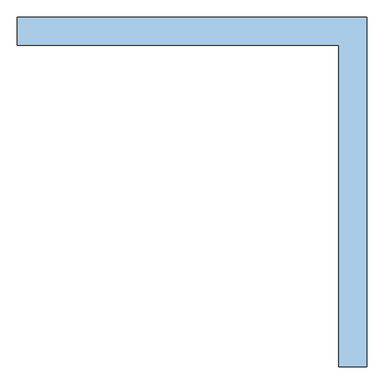
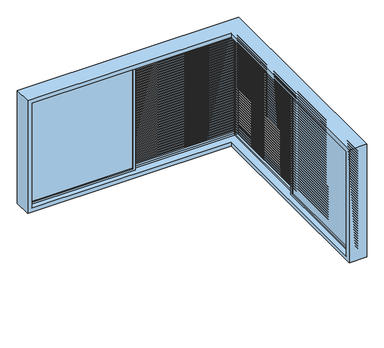
"""IFC4 building model written with IfcOpenShell, lengths in millimetres: window geometry, .CC_ND 300_JANELA DE CANTO_6 FOLHAS DE CORRER_VENEZIANA_VIDRO : 2.50F X 2.50E X 1.35H."""

from ifc_helpers import new_model, si_unit, frame, origin, place, context, project, spatial, polyline, outline, extrude, faceted_brep, source, transform, mapped, element, save


def window_869adda8(model_context):
    return source(origin(), model_context, "Body", "SolidModel", [
        extrude(outline(polyline([(2110.1282051, 1161.2), (2110.1282051, 1166.2), (2145.1282051, 1141.2), (2145.1282051, 1136.2), (2110.1282051, 1161.2)])), frame((0.0, -1170.6, 0.0), z_axis=(0.0, 1.0, 0.0), x_axis=(0.0, 0.0, 1.0)), (0.0, 0.0, 1.0), 1130.6),
        extrude(outline(polyline([(2080.2564103, 1161.2), (2080.2564103, 1166.2), (2115.2564103, 1141.2), (2115.2564103, 1136.2), (2080.2564103, 1161.2)])), frame((0.0, -1170.6, 0.0), z_axis=(0.0, 1.0, 0.0), x_axis=(0.0, 0.0, 1.0)), (0.0, 0.0, 1.0), 1130.6),
        extrude(outline(polyline([(2050.3846154, 1161.2), (2050.3846154, 1166.2), (2085.3846154, 1141.2), (2085.3846154, 1136.2), (2050.3846154, 1161.2)])), frame((0.0, -1170.6, 0.0), z_axis=(0.0, 1.0, 0.0), x_axis=(0.0, 0.0, 1.0)), (0.0, 0.0, 1.0), 1130.6),
        extrude(outline(polyline([(2020.5128205, 1161.2), (2020.5128205, 1166.2), (2055.5128205, 1141.2), (2055.5128205, 1136.2), (2020.5128205, 1161.2)])), frame((0.0, -1170.6, 0.0), z_axis=(0.0, 1.0, 0.0), x_axis=(0.0, 0.0, 1.0)), (0.0, 0.0, 1.0), 1130.6),
        extrude(outline(polyline([(1990.6410256, 1161.2), (1990.6410256, 1166.2), (2025.6410256, 1141.2), (2025.6410256, 1136.2), (1990.6410256, 1161.2)])), frame((0.0, -1170.6, 0.0), z_axis=(0.0, 1.0, 0.0), x_axis=(0.0, 0.0, 1.0)), (0.0, 0.0, 1.0), 1130.6),
        extrude(outline(polyline([(1960.7692308, 1161.2), (1960.7692308, 1166.2), (1995.7692308, 1141.2), (1995.7692308, 1136.2), (1960.7692308, 1161.2)])), frame((0.0, -1170.6, 0.0), z_axis=(0.0, 1.0, 0.0), x_axis=(0.0, 0.0, 1.0)), (0.0, 0.0, 1.0), 1130.6),
        extrude(outline(polyline([(1930.8974359, 1161.2), (1930.8974359, 1166.2), (1965.8974359, 1141.2), (1965.8974359, 1136.2), (1930.8974359, 1161.2)])), frame((0.0, -1170.6, 0.0), z_axis=(0.0, 1.0, 0.0), x_axis=(0.0, 0.0, 1.0)), (0.0, 0.0, 1.0), 1130.6),
        extrude(outline(polyline([(1901.025641, 1161.2), (1901.025641, 1166.2), (1936.025641, 1141.2), (1936.025641, 1136.2), (1901.025641, 1161.2)])), frame((0.0, -1170.6, 0.0), z_axis=(0.0, 1.0, 0.0), x_axis=(0.0, 0.0, 1.0)), (0.0, 0.0, 1.0), 1130.6),
        extrude(outline(polyline([(1871.1538462, 1161.2), (1871.1538462, 1166.2), (1906.1538462, 1141.2), (1906.1538462, 1136.2), (1871.1538462, 1161.2)])), frame((0.0, -1170.6, 0.0), z_axis=(0.0, 1.0, 0.0), x_axis=(0.0, 0.0, 1.0)), (0.0, 0.0, 1.0), 1130.6),
        extrude(outline(polyline([(1841.2820513, 1161.2), (1841.2820513, 1166.2), (1876.2820513, 1141.2), (1876.2820513, 1136.2), (1841.2820513, 1161.2)])), frame((0.0, -1170.6, 0.0), z_axis=(0.0, 1.0, 0.0), x_axis=(0.0, 0.0, 1.0)), (0.0, 0.0, 1.0), 1130.6),
        extrude(outline(polyline([(1811.4102564, 1161.2), (1811.4102564, 1166.2), (1846.4102564, 1141.2), (1846.4102564, 1136.2), (1811.4102564, 1161.2)])), frame((0.0, -1170.6, 0.0), z_axis=(0.0, 1.0, 0.0), x_axis=(0.0, 0.0, 1.0)), (0.0, 0.0, 1.0), 1130.6),
        extrude(outline(polyline([(1781.5384615, 1161.2), (1781.5384615, 1166.2), (1816.5384615, 1141.2), (1816.5384615, 1136.2), (1781.5384615, 1161.2)])), frame((0.0, -1170.6, 0.0), z_axis=(0.0, 1.0, 0.0), x_axis=(0.0, 0.0, 1.0)), (0.0, 0.0, 1.0), 1130.6),
        extrude(outline(polyline([(1751.6666667, 1161.2), (1751.6666667, 1166.2), (1786.6666667, 1141.2), (1786.6666667, 1136.2), (1751.6666667, 1161.2)])), frame((0.0, -1170.6, 0.0), z_axis=(0.0, 1.0, 0.0), x_axis=(0.0, 0.0, 1.0)), (0.0, 0.0, 1.0), 1130.6),
        extrude(outline(polyline([(1721.7948718, 1161.2), (1721.7948718, 1166.2), (1756.7948718, 1141.2), (1756.7948718, 1136.2), (1721.7948718, 1161.2)])), frame((0.0, -1170.6, 0.0), z_axis=(0.0, 1.0, 0.0), x_axis=(0.0, 0.0, 1.0)), (0.0, 0.0, 1.0), 1130.6),
        extrude(outline(polyline([(1691.9230769, 1161.2), (1691.9230769, 1166.2), (1726.9230769, 1141.2), (1726.9230769, 1136.2), (1691.9230769, 1161.2)])), frame((0.0, -1170.6, 0.0), z_axis=(0.0, 1.0, 0.0), x_axis=(0.0, 0.0, 1.0)), (0.0, 0.0, 1.0), 1130.6),
        extrude(outline(polyline([(1662.0512821, 1161.2), (1662.0512821, 1166.2), (1697.0512821, 1141.2), (1697.0512821, 1136.2), (1662.0512821, 1161.2)])), frame((0.0, -1170.6, 0.0), z_axis=(0.0, 1.0, 0.0), x_axis=(0.0, 0.0, 1.0)), (0.0, 0.0, 1.0), 1130.6),
        extrude(outline(polyline([(1632.1794872, 1161.2), (1632.1794872, 1166.2), (1667.1794872, 1141.2), (1667.1794872, 1136.2), (1632.1794872, 1161.2)])), frame((0.0, -1170.6, 0.0), z_axis=(0.0, 1.0, 0.0), x_axis=(0.0, 0.0, 1.0)), (0.0, 0.0, 1.0), 1130.6),
        extrude(outline(polyline([(1602.3076923, 1161.2), (1602.3076923, 1166.2), (1637.3076923, 1141.2), (1637.3076923, 1136.2), (1602.3076923, 1161.2)])), frame((0.0, -1170.6, 0.0), z_axis=(0.0, 1.0, 0.0), x_axis=(0.0, 0.0, 1.0)), (0.0, 0.0, 1.0), 1130.6),
        extrude(outline(polyline([(1572.4358974, 1161.2), (1572.4358974, 1166.2), (1607.4358974, 1141.2), (1607.4358974, 1136.2), (1572.4358974, 1161.2)])), frame((0.0, -1170.6, 0.0), z_axis=(0.0, 1.0, 0.0), x_axis=(0.0, 0.0, 1.0)), (0.0, 0.0, 1.0), 1130.6),
        extrude(outline(polyline([(1542.5641026, 1161.2), (1542.5641026, 1166.2), (1577.5641026, 1141.2), (1577.5641026, 1136.2), (1542.5641026, 1161.2)])), frame((0.0, -1170.6, 0.0), z_axis=(0.0, 1.0, 0.0), x_axis=(0.0, 0.0, 1.0)), (0.0, 0.0, 1.0), 1130.6),
        extrude(outline(polyline([(1512.6923077, 1161.2), (1512.6923077, 1166.2), (1547.6923077, 1141.2), (1547.6923077, 1136.2), (1512.6923077, 1161.2)])), frame((0.0, -1170.6, 0.0), z_axis=(0.0, 1.0, 0.0), x_axis=(0.0, 0.0, 1.0)), (0.0, 0.0, 1.0), 1130.6),
        extrude(outline(polyline([(1482.8205128, 1161.2), (1482.8205128, 1166.2), (1517.8205128, 1141.2), (1517.8205128, 1136.2), (1482.8205128, 1161.2)])), frame((0.0, -1170.6, 0.0), z_axis=(0.0, 1.0, 0.0), x_axis=(0.0, 0.0, 1.0)), (0.0, 0.0, 1.0), 1130.6),
        extrude(outline(polyline([(1452.9487179, 1161.2), (1452.9487179, 1166.2), (1487.9487179, 1141.2), (1487.9487179, 1136.2), (1452.9487179, 1161.2)])), frame((0.0, -1170.6, 0.0), z_axis=(0.0, 1.0, 0.0), x_axis=(0.0, 0.0, 1.0)), (0.0, 0.0, 1.0), 1130.6),
        extrude(outline(polyline([(1423.0769231, 1161.2), (1423.0769231, 1166.2), (1458.0769231, 1141.2), (1458.0769231, 1136.2), (1423.0769231, 1161.2)])), frame((0.0, -1170.6, 0.0), z_axis=(0.0, 1.0, 0.0), x_axis=(0.0, 0.0, 1.0)), (0.0, 0.0, 1.0), 1130.6),
        extrude(outline(polyline([(1393.2051282, 1161.2), (1393.2051282, 1166.2), (1428.2051282, 1141.2), (1428.2051282, 1136.2), (1393.2051282, 1161.2)])), frame((0.0, -1170.6, 0.0), z_axis=(0.0, 1.0, 0.0), x_axis=(0.0, 0.0, 1.0)), (0.0, 0.0, 1.0), 1130.6),
        extrude(outline(polyline([(1363.3333333, 1161.2), (1363.3333333, 1166.2), (1398.3333333, 1141.2), (1398.3333333, 1136.2), (1363.3333333, 1161.2)])), frame((0.0, -1170.6, 0.0), z_axis=(0.0, 1.0, 0.0), x_axis=(0.0, 0.0, 1.0)), (0.0, 0.0, 1.0), 1130.6),
        extrude(outline(polyline([(1333.4615385, 1161.2), (1333.4615385, 1166.2), (1368.4615385, 1141.2), (1368.4615385, 1136.2), (1333.4615385, 1161.2)])), frame((0.0, -1170.6, 0.0), z_axis=(0.0, 1.0, 0.0), x_axis=(0.0, 0.0, 1.0)), (0.0, 0.0, 1.0), 1130.6),
        extrude(outline(polyline([(1303.5897436, 1161.2), (1303.5897436, 1166.2), (1338.5897436, 1141.2), (1338.5897436, 1136.2), (1303.5897436, 1161.2)])), frame((0.0, -1170.6, 0.0), z_axis=(0.0, 1.0, 0.0), x_axis=(0.0, 0.0, 1.0)), (0.0, 0.0, 1.0), 1130.6),
        extrude(outline(polyline([(1273.7179487, 1161.2), (1273.7179487, 1166.2), (1308.7179487, 1141.2), (1308.7179487, 1136.2), (1273.7179487, 1161.2)])), frame((0.0, -1170.6, 0.0), z_axis=(0.0, 1.0, 0.0), x_axis=(0.0, 0.0, 1.0)), (0.0, 0.0, 1.0), 1130.6),
        extrude(outline(polyline([(1243.8461538, 1161.2), (1243.8461538, 1166.2), (1278.8461538, 1141.2), (1278.8461538, 1136.2), (1243.8461538, 1161.2)])), frame((0.0, -1170.6, 0.0), z_axis=(0.0, 1.0, 0.0), x_axis=(0.0, 0.0, 1.0)), (0.0, 0.0, 1.0), 1130.6),
        extrude(outline(polyline([(1213.974359, 1161.2), (1213.974359, 1166.2), (1248.974359, 1141.2), (1248.974359, 1136.2), (1213.974359, 1161.2)])), frame((0.0, -1170.6, 0.0), z_axis=(0.0, 1.0, 0.0), x_axis=(0.0, 0.0, 1.0)), (0.0, 0.0, 1.0), 1130.6),
        extrude(outline(polyline([(1184.1025641, 1161.2), (1184.1025641, 1166.2), (1219.1025641, 1141.2), (1219.1025641, 1136.2), (1184.1025641, 1161.2)])), frame((0.0, -1170.6, 0.0), z_axis=(0.0, 1.0, 0.0), x_axis=(0.0, 0.0, 1.0)), (0.0, 0.0, 1.0), 1130.6),
        extrude(outline(polyline([(1154.2307692, 1161.2), (1154.2307692, 1166.2), (1189.2307692, 1141.2), (1189.2307692, 1136.2), (1154.2307692, 1161.2)])), frame((0.0, -1170.6, 0.0), z_axis=(0.0, 1.0, 0.0), x_axis=(0.0, 0.0, 1.0)), (0.0, 0.0, 1.0), 1130.6),
        extrude(outline(polyline([(1124.3589744, 1161.2), (1124.3589744, 1166.2), (1159.3589744, 1141.2), (1159.3589744, 1136.2), (1124.3589744, 1161.2)])), frame((0.0, -1170.6, 0.0), z_axis=(0.0, 1.0, 0.0), x_axis=(0.0, 0.0, 1.0)), (0.0, 0.0, 1.0), 1130.6),
        extrude(outline(polyline([(1094.4871795, 1161.2), (1094.4871795, 1166.2), (1129.4871795, 1141.2), (1129.4871795, 1136.2), (1094.4871795, 1161.2)])), frame((0.0, -1170.6, 0.0), z_axis=(0.0, 1.0, 0.0), x_axis=(0.0, 0.0, 1.0)), (0.0, 0.0, 1.0), 1130.6),
        extrude(outline(polyline([(1064.6153846, 1161.2), (1064.6153846, 1166.2), (1099.6153846, 1141.2), (1099.6153846, 1136.2), (1064.6153846, 1161.2)])), frame((0.0, -1170.6, 0.0), z_axis=(0.0, 1.0, 0.0), x_axis=(0.0, 0.0, 1.0)), (0.0, 0.0, 1.0), 1130.6),
        extrude(outline(polyline([(1034.7435897, 1161.2), (1034.7435897, 1166.2), (1069.7435897, 1141.2), (1069.7435897, 1136.2), (1034.7435897, 1161.2)])), frame((0.0, -1170.6, 0.0), z_axis=(0.0, 1.0, 0.0), x_axis=(0.0, 0.0, 1.0)), (0.0, 0.0, 1.0), 1130.6),
        extrude(outline(polyline([(1004.8717949, 1161.2), (1004.8717949, 1166.2), (1039.8717949, 1141.2), (1039.8717949, 1136.2), (1004.8717949, 1161.2)])), frame((0.0, -1170.6, 0.0), z_axis=(0.0, 1.0, 0.0), x_axis=(0.0, 0.0, 1.0)), (0.0, 0.0, 1.0), 1130.6),
        extrude(outline(polyline([(2140.0, 1161.2), (2140.0, 1166.2), (2175.0, 1141.2), (2175.0, 1136.2), (2140.0, 1161.2)])), frame((0.0, -1170.6, 0.0), z_axis=(0.0, 1.0, 0.0), x_axis=(0.0, 0.0, 1.0)), (0.0, 0.0, 1.0), 1130.6),
        extrude(outline(polyline([(975.0, 1161.2), (975.0, 1166.2), (1010.0, 1141.2), (1010.0, 1136.2), (975.0, 1161.2)])), frame((0.0, -1170.6, 0.0), z_axis=(0.0, 1.0, 0.0), x_axis=(0.0, 0.0, 1.0)), (0.0, 0.0, 1.0), 1130.6),
        extrude(outline(polyline([(-15.0, 2200.0), (-15.0, 950.0), (-1195.6, 950.0), (-1195.6, 2200.0), (-15.0, 2200.0)]), holes=[polyline([(-40.0, 2175.0), (-1170.6, 2175.0), (-1170.6, 975.0), (-40.0, 975.0), (-40.0, 2175.0)])]), frame((1136.2, 0.0, 0.0), z_axis=(1.0, 0.0, 0.0), x_axis=(0.0, 1.0, 0.0)), (0.0, 0.0, 1.0), 30.0),
        extrude(outline(polyline([(2110.1282051, 1191.2), (2110.1282051, 1196.2), (2145.1282051, 1171.2), (2145.1282051, 1166.2), (2110.1282051, 1191.2)])), frame((0.0, -2326.2, 0.0), z_axis=(0.0, 1.0, 0.0), x_axis=(0.0, 0.0, 1.0)), (0.0, 0.0, 1.0), 1130.6),
        extrude(outline(polyline([(2080.2564103, 1191.2), (2080.2564103, 1196.2), (2115.2564103, 1171.2), (2115.2564103, 1166.2), (2080.2564103, 1191.2)])), frame((0.0, -2326.2, 0.0), z_axis=(0.0, 1.0, 0.0), x_axis=(0.0, 0.0, 1.0)), (0.0, 0.0, 1.0), 1130.6),
        extrude(outline(polyline([(2050.3846154, 1191.2), (2050.3846154, 1196.2), (2085.3846154, 1171.2), (2085.3846154, 1166.2), (2050.3846154, 1191.2)])), frame((0.0, -2326.2, 0.0), z_axis=(0.0, 1.0, 0.0), x_axis=(0.0, 0.0, 1.0)), (0.0, 0.0, 1.0), 1130.6),
        extrude(outline(polyline([(2020.5128205, 1191.2), (2020.5128205, 1196.2), (2055.5128205, 1171.2), (2055.5128205, 1166.2), (2020.5128205, 1191.2)])), frame((0.0, -2326.2, 0.0), z_axis=(0.0, 1.0, 0.0), x_axis=(0.0, 0.0, 1.0)), (0.0, 0.0, 1.0), 1130.6),
        extrude(outline(polyline([(1990.6410256, 1191.2), (1990.6410256, 1196.2), (2025.6410256, 1171.2), (2025.6410256, 1166.2), (1990.6410256, 1191.2)])), frame((0.0, -2326.2, 0.0), z_axis=(0.0, 1.0, 0.0), x_axis=(0.0, 0.0, 1.0)), (0.0, 0.0, 1.0), 1130.6),
        extrude(outline(polyline([(1960.7692308, 1191.2), (1960.7692308, 1196.2), (1995.7692308, 1171.2), (1995.7692308, 1166.2), (1960.7692308, 1191.2)])), frame((0.0, -2326.2, 0.0), z_axis=(0.0, 1.0, 0.0), x_axis=(0.0, 0.0, 1.0)), (0.0, 0.0, 1.0), 1130.6),
        extrude(outline(polyline([(1930.8974359, 1191.2), (1930.8974359, 1196.2), (1965.8974359, 1171.2), (1965.8974359, 1166.2), (1930.8974359, 1191.2)])), frame((0.0, -2326.2, 0.0), z_axis=(0.0, 1.0, 0.0), x_axis=(0.0, 0.0, 1.0)), (0.0, 0.0, 1.0), 1130.6),
        extrude(outline(polyline([(1901.025641, 1191.2), (1901.025641, 1196.2), (1936.025641, 1171.2), (1936.025641, 1166.2), (1901.025641, 1191.2)])), frame((0.0, -2326.2, 0.0), z_axis=(0.0, 1.0, 0.0), x_axis=(0.0, 0.0, 1.0)), (0.0, 0.0, 1.0), 1130.6),
        extrude(outline(polyline([(1871.1538462, 1191.2), (1871.1538462, 1196.2), (1906.1538462, 1171.2), (1906.1538462, 1166.2), (1871.1538462, 1191.2)])), frame((0.0, -2326.2, 0.0), z_axis=(0.0, 1.0, 0.0), x_axis=(0.0, 0.0, 1.0)), (0.0, 0.0, 1.0), 1130.6),
        extrude(outline(polyline([(1841.2820513, 1191.2), (1841.2820513, 1196.2), (1876.2820513, 1171.2), (1876.2820513, 1166.2), (1841.2820513, 1191.2)])), frame((0.0, -2326.2, 0.0), z_axis=(0.0, 1.0, 0.0), x_axis=(0.0, 0.0, 1.0)), (0.0, 0.0, 1.0), 1130.6),
        extrude(outline(polyline([(1811.4102564, 1191.2), (1811.4102564, 1196.2), (1846.4102564, 1171.2), (1846.4102564, 1166.2), (1811.4102564, 1191.2)])), frame((0.0, -2326.2, 0.0), z_axis=(0.0, 1.0, 0.0), x_axis=(0.0, 0.0, 1.0)), (0.0, 0.0, 1.0), 1130.6),
        extrude(outline(polyline([(1781.5384615, 1191.2), (1781.5384615, 1196.2), (1816.5384615, 1171.2), (1816.5384615, 1166.2), (1781.5384615, 1191.2)])), frame((0.0, -2326.2, 0.0), z_axis=(0.0, 1.0, 0.0), x_axis=(0.0, 0.0, 1.0)), (0.0, 0.0, 1.0), 1130.6),
        extrude(outline(polyline([(1751.6666667, 1191.2), (1751.6666667, 1196.2), (1786.6666667, 1171.2), (1786.6666667, 1166.2), (1751.6666667, 1191.2)])), frame((0.0, -2326.2, 0.0), z_axis=(0.0, 1.0, 0.0), x_axis=(0.0, 0.0, 1.0)), (0.0, 0.0, 1.0), 1130.6),
        extrude(outline(polyline([(1721.7948718, 1191.2), (1721.7948718, 1196.2), (1756.7948718, 1171.2), (1756.7948718, 1166.2), (1721.7948718, 1191.2)])), frame((0.0, -2326.2, 0.0), z_axis=(0.0, 1.0, 0.0), x_axis=(0.0, 0.0, 1.0)), (0.0, 0.0, 1.0), 1130.6),
        extrude(outline(polyline([(1691.9230769, 1191.2), (1691.9230769, 1196.2), (1726.9230769, 1171.2), (1726.9230769, 1166.2), (1691.9230769, 1191.2)])), frame((0.0, -2326.2, 0.0), z_axis=(0.0, 1.0, 0.0), x_axis=(0.0, 0.0, 1.0)), (0.0, 0.0, 1.0), 1130.6),
        extrude(outline(polyline([(1662.0512821, 1191.2), (1662.0512821, 1196.2), (1697.0512821, 1171.2), (1697.0512821, 1166.2), (1662.0512821, 1191.2)])), frame((0.0, -2326.2, 0.0), z_axis=(0.0, 1.0, 0.0), x_axis=(0.0, 0.0, 1.0)), (0.0, 0.0, 1.0), 1130.6),
        extrude(outline(polyline([(1632.1794872, 1191.2), (1632.1794872, 1196.2), (1667.1794872, 1171.2), (1667.1794872, 1166.2), (1632.1794872, 1191.2)])), frame((0.0, -2326.2, 0.0), z_axis=(0.0, 1.0, 0.0), x_axis=(0.0, 0.0, 1.0)), (0.0, 0.0, 1.0), 1130.6),
        extrude(outline(polyline([(1602.3076923, 1191.2), (1602.3076923, 1196.2), (1637.3076923, 1171.2), (1637.3076923, 1166.2), (1602.3076923, 1191.2)])), frame((0.0, -2326.2, 0.0), z_axis=(0.0, 1.0, 0.0), x_axis=(0.0, 0.0, 1.0)), (0.0, 0.0, 1.0), 1130.6),
        extrude(outline(polyline([(1572.4358974, 1191.2), (1572.4358974, 1196.2), (1607.4358974, 1171.2), (1607.4358974, 1166.2), (1572.4358974, 1191.2)])), frame((0.0, -2326.2, 0.0), z_axis=(0.0, 1.0, 0.0), x_axis=(0.0, 0.0, 1.0)), (0.0, 0.0, 1.0), 1130.6),
        extrude(outline(polyline([(1542.5641026, 1191.2), (1542.5641026, 1196.2), (1577.5641026, 1171.2), (1577.5641026, 1166.2), (1542.5641026, 1191.2)])), frame((0.0, -2326.2, 0.0), z_axis=(0.0, 1.0, 0.0), x_axis=(0.0, 0.0, 1.0)), (0.0, 0.0, 1.0), 1130.6),
        extrude(outline(polyline([(1512.6923077, 1191.2), (1512.6923077, 1196.2), (1547.6923077, 1171.2), (1547.6923077, 1166.2), (1512.6923077, 1191.2)])), frame((0.0, -2326.2, 0.0), z_axis=(0.0, 1.0, 0.0), x_axis=(0.0, 0.0, 1.0)), (0.0, 0.0, 1.0), 1130.6),
        extrude(outline(polyline([(1482.8205128, 1191.2), (1482.8205128, 1196.2), (1517.8205128, 1171.2), (1517.8205128, 1166.2), (1482.8205128, 1191.2)])), frame((0.0, -2326.2, 0.0), z_axis=(0.0, 1.0, 0.0), x_axis=(0.0, 0.0, 1.0)), (0.0, 0.0, 1.0), 1130.6),
        extrude(outline(polyline([(1452.9487179, 1191.2), (1452.9487179, 1196.2), (1487.9487179, 1171.2), (1487.9487179, 1166.2), (1452.9487179, 1191.2)])), frame((0.0, -2326.2, 0.0), z_axis=(0.0, 1.0, 0.0), x_axis=(0.0, 0.0, 1.0)), (0.0, 0.0, 1.0), 1130.6),
        extrude(outline(polyline([(1423.0769231, 1191.2), (1423.0769231, 1196.2), (1458.0769231, 1171.2), (1458.0769231, 1166.2), (1423.0769231, 1191.2)])), frame((0.0, -2326.2, 0.0), z_axis=(0.0, 1.0, 0.0), x_axis=(0.0, 0.0, 1.0)), (0.0, 0.0, 1.0), 1130.6),
        extrude(outline(polyline([(1393.2051282, 1191.2), (1393.2051282, 1196.2), (1428.2051282, 1171.2), (1428.2051282, 1166.2), (1393.2051282, 1191.2)])), frame((0.0, -2326.2, 0.0), z_axis=(0.0, 1.0, 0.0), x_axis=(0.0, 0.0, 1.0)), (0.0, 0.0, 1.0), 1130.6),
        extrude(outline(polyline([(1363.3333333, 1191.2), (1363.3333333, 1196.2), (1398.3333333, 1171.2), (1398.3333333, 1166.2), (1363.3333333, 1191.2)])), frame((0.0, -2326.2, 0.0), z_axis=(0.0, 1.0, 0.0), x_axis=(0.0, 0.0, 1.0)), (0.0, 0.0, 1.0), 1130.6),
        extrude(outline(polyline([(1333.4615385, 1191.2), (1333.4615385, 1196.2), (1368.4615385, 1171.2), (1368.4615385, 1166.2), (1333.4615385, 1191.2)])), frame((0.0, -2326.2, 0.0), z_axis=(0.0, 1.0, 0.0), x_axis=(0.0, 0.0, 1.0)), (0.0, 0.0, 1.0), 1130.6),
        extrude(outline(polyline([(1303.5897436, 1191.2), (1303.5897436, 1196.2), (1338.5897436, 1171.2), (1338.5897436, 1166.2), (1303.5897436, 1191.2)])), frame((0.0, -2326.2, 0.0), z_axis=(0.0, 1.0, 0.0), x_axis=(0.0, 0.0, 1.0)), (0.0, 0.0, 1.0), 1130.6),
        extrude(outline(polyline([(1273.7179487, 1191.2), (1273.7179487, 1196.2), (1308.7179487, 1171.2), (1308.7179487, 1166.2), (1273.7179487, 1191.2)])), frame((0.0, -2326.2, 0.0), z_axis=(0.0, 1.0, 0.0), x_axis=(0.0, 0.0, 1.0)), (0.0, 0.0, 1.0), 1130.6),
        extrude(outline(polyline([(1243.8461538, 1191.2), (1243.8461538, 1196.2), (1278.8461538, 1171.2), (1278.8461538, 1166.2), (1243.8461538, 1191.2)])), frame((0.0, -2326.2, 0.0), z_axis=(0.0, 1.0, 0.0), x_axis=(0.0, 0.0, 1.0)), (0.0, 0.0, 1.0), 1130.6),
        extrude(outline(polyline([(1213.974359, 1191.2), (1213.974359, 1196.2), (1248.974359, 1171.2), (1248.974359, 1166.2), (1213.974359, 1191.2)])), frame((0.0, -2326.2, 0.0), z_axis=(0.0, 1.0, 0.0), x_axis=(0.0, 0.0, 1.0)), (0.0, 0.0, 1.0), 1130.6),
        extrude(outline(polyline([(1184.1025641, 1191.2), (1184.1025641, 1196.2), (1219.1025641, 1171.2), (1219.1025641, 1166.2), (1184.1025641, 1191.2)])), frame((0.0, -2326.2, 0.0), z_axis=(0.0, 1.0, 0.0), x_axis=(0.0, 0.0, 1.0)), (0.0, 0.0, 1.0), 1130.6),
        extrude(outline(polyline([(1154.2307692, 1191.2), (1154.2307692, 1196.2), (1189.2307692, 1171.2), (1189.2307692, 1166.2), (1154.2307692, 1191.2)])), frame((0.0, -2326.2, 0.0), z_axis=(0.0, 1.0, 0.0), x_axis=(0.0, 0.0, 1.0)), (0.0, 0.0, 1.0), 1130.6),
        extrude(outline(polyline([(1124.3589744, 1191.2), (1124.3589744, 1196.2), (1159.3589744, 1171.2), (1159.3589744, 1166.2), (1124.3589744, 1191.2)])), frame((0.0, -2326.2, 0.0), z_axis=(0.0, 1.0, 0.0), x_axis=(0.0, 0.0, 1.0)), (0.0, 0.0, 1.0), 1130.6),
        extrude(outline(polyline([(1094.4871795, 1191.2), (1094.4871795, 1196.2), (1129.4871795, 1171.2), (1129.4871795, 1166.2), (1094.4871795, 1191.2)])), frame((0.0, -2326.2, 0.0), z_axis=(0.0, 1.0, 0.0), x_axis=(0.0, 0.0, 1.0)), (0.0, 0.0, 1.0), 1130.6),
        extrude(outline(polyline([(1064.6153846, 1191.2), (1064.6153846, 1196.2), (1099.6153846, 1171.2), (1099.6153846, 1166.2), (1064.6153846, 1191.2)])), frame((0.0, -2326.2, 0.0), z_axis=(0.0, 1.0, 0.0), x_axis=(0.0, 0.0, 1.0)), (0.0, 0.0, 1.0), 1130.6),
        extrude(outline(polyline([(1034.7435897, 1191.2), (1034.7435897, 1196.2), (1069.7435897, 1171.2), (1069.7435897, 1166.2), (1034.7435897, 1191.2)])), frame((0.0, -2326.2, 0.0), z_axis=(0.0, 1.0, 0.0), x_axis=(0.0, 0.0, 1.0)), (0.0, 0.0, 1.0), 1130.6),
        extrude(outline(polyline([(1004.8717949, 1191.2), (1004.8717949, 1196.2), (1039.8717949, 1171.2), (1039.8717949, 1166.2), (1004.8717949, 1191.2)])), frame((0.0, -2326.2, 0.0), z_axis=(0.0, 1.0, 0.0), x_axis=(0.0, 0.0, 1.0)), (0.0, 0.0, 1.0), 1130.6),
        extrude(outline(polyline([(2140.0, 1191.2), (2140.0, 1196.2), (2175.0, 1171.2), (2175.0, 1166.2), (2140.0, 1191.2)])), frame((0.0, -2326.2, 0.0), z_axis=(0.0, 1.0, 0.0), x_axis=(0.0, 0.0, 1.0)), (0.0, 0.0, 1.0), 1130.6),
        extrude(outline(polyline([(975.0, 1191.2), (975.0, 1196.2), (1010.0, 1171.2), (1010.0, 1166.2), (975.0, 1191.2)])), frame((0.0, -2326.2, 0.0), z_axis=(0.0, 1.0, 0.0), x_axis=(0.0, 0.0, 1.0)), (0.0, 0.0, 1.0), 1130.6),
        extrude(outline(polyline([(-1170.6, 2200.0), (-1170.6, 950.0), (-2351.2, 950.0), (-2351.2, 2200.0), (-1170.6, 2200.0)]), holes=[polyline([(-1195.6, 2175.0), (-2326.2, 2175.0), (-2326.2, 975.0), (-1195.6, 975.0), (-1195.6, 2175.0)])]), frame((1166.2, 0.0, 0.0), z_axis=(1.0, 0.0, 0.0), x_axis=(0.0, 1.0, 0.0)), (0.0, 0.0, 1.0), 30.0),
        extrude(outline(polyline([(-1170.6, 2200.0), (-1170.6, 950.0), (-2351.2, 950.0), (-2351.2, 2200.0), (-1170.6, 2200.0)]), holes=[polyline([(-1195.6, 2175.0), (-2326.2, 2175.0), (-2326.2, 975.0), (-1195.6, 975.0), (-1195.6, 2175.0)])]), frame((1106.2, 0.0, 0.0), z_axis=(1.0, 0.0, 0.0), x_axis=(0.0, 1.0, 0.0)), (0.0, 0.0, 1.0), 30.0),
        extrude(outline(polyline([(1117.2, -1195.6), (1125.2, -1195.6), (1125.2, -2326.2), (1117.2, -2326.2), (1117.2, -1195.6)])), frame((0.0, 0.0, 975.0), z_axis=(0.0, 0.0, 1.0), x_axis=(1.0, 0.0, 0.0)), (0.0, 0.0, 1.0), 1200.0),
        extrude(outline(polyline([(2200.0, -4.4), (2200.0, -1200.0), (950.0, -1200.0), (950.0, -4.4), (2200.0, -4.4)]), holes=[polyline([(2175.0, -29.4), (975.0, -29.4), (975.0, -1175.0), (2175.0, -1175.0), (2175.0, -29.4)])]), frame((0.0, -45.0, 0.0), z_axis=(0.0, 1.0, 0.0), x_axis=(0.0, 0.0, 1.0)), (0.0, 0.0, 1.0), 30.0),
        extrude(outline(polyline([(-29.4, -26.0), (-29.4, -34.0), (-1175.0, -34.0), (-1175.0, -26.0), (-29.4, -26.0)])), frame((0.0, 0.0, 975.0), z_axis=(0.0, 0.0, 1.0), x_axis=(1.0, 0.0, 0.0)), (0.0, 0.0, 1.0), 1200.0),
        extrude(outline(polyline([(10.0, 2110.1282051), (-15.0, 2145.1282051), (-10.0, 2145.1282051), (15.0, 2110.1282051), (10.0, 2110.1282051)])), frame((-4.4, 0.0, 0.0), z_axis=(1.0, 0.0, 0.0), x_axis=(0.0, 1.0, 0.0)), (0.0, 0.0, 1.0), 1145.6),
        extrude(outline(polyline([(10.0, 2080.2564103), (-15.0, 2115.2564103), (-10.0, 2115.2564103), (15.0, 2080.2564103), (10.0, 2080.2564103)])), frame((-4.4, 0.0, 0.0), z_axis=(1.0, 0.0, 0.0), x_axis=(0.0, 1.0, 0.0)), (0.0, 0.0, 1.0), 1145.6),
        extrude(outline(polyline([(10.0, 2050.3846154), (-15.0, 2085.3846154), (-10.0, 2085.3846154), (15.0, 2050.3846154), (10.0, 2050.3846154)])), frame((-4.4, 0.0, 0.0), z_axis=(1.0, 0.0, 0.0), x_axis=(0.0, 1.0, 0.0)), (0.0, 0.0, 1.0), 1145.6),
        extrude(outline(polyline([(10.0, 2020.5128205), (-15.0, 2055.5128205), (-10.0, 2055.5128205), (15.0, 2020.5128205), (10.0, 2020.5128205)])), frame((-4.4, 0.0, 0.0), z_axis=(1.0, 0.0, 0.0), x_axis=(0.0, 1.0, 0.0)), (0.0, 0.0, 1.0), 1145.6),
        extrude(outline(polyline([(10.0, 1990.6410256), (-15.0, 2025.6410256), (-10.0, 2025.6410256), (15.0, 1990.6410256), (10.0, 1990.6410256)])), frame((-4.4, 0.0, 0.0), z_axis=(1.0, 0.0, 0.0), x_axis=(0.0, 1.0, 0.0)), (0.0, 0.0, 1.0), 1145.6),
        extrude(outline(polyline([(10.0, 1960.7692308), (-15.0, 1995.7692308), (-10.0, 1995.7692308), (15.0, 1960.7692308), (10.0, 1960.7692308)])), frame((-4.4, 0.0, 0.0), z_axis=(1.0, 0.0, 0.0), x_axis=(0.0, 1.0, 0.0)), (0.0, 0.0, 1.0), 1145.6),
        extrude(outline(polyline([(10.0, 1930.8974359), (-15.0, 1965.8974359), (-10.0, 1965.8974359), (15.0, 1930.8974359), (10.0, 1930.8974359)])), frame((-4.4, 0.0, 0.0), z_axis=(1.0, 0.0, 0.0), x_axis=(0.0, 1.0, 0.0)), (0.0, 0.0, 1.0), 1145.6),
        extrude(outline(polyline([(10.0, 1901.025641), (-15.0, 1936.025641), (-10.0, 1936.025641), (15.0, 1901.025641), (10.0, 1901.025641)])), frame((-4.4, 0.0, 0.0), z_axis=(1.0, 0.0, 0.0), x_axis=(0.0, 1.0, 0.0)), (0.0, 0.0, 1.0), 1145.6),
        extrude(outline(polyline([(10.0, 1871.1538462), (-15.0, 1906.1538462), (-10.0, 1906.1538462), (15.0, 1871.1538462), (10.0, 1871.1538462)])), frame((-4.4, 0.0, 0.0), z_axis=(1.0, 0.0, 0.0), x_axis=(0.0, 1.0, 0.0)), (0.0, 0.0, 1.0), 1145.6),
        extrude(outline(polyline([(10.0, 1841.2820513), (-15.0, 1876.2820513), (-10.0, 1876.2820513), (15.0, 1841.2820513), (10.0, 1841.2820513)])), frame((-4.4, 0.0, 0.0), z_axis=(1.0, 0.0, 0.0), x_axis=(0.0, 1.0, 0.0)), (0.0, 0.0, 1.0), 1145.6),
        extrude(outline(polyline([(10.0, 1811.4102564), (-15.0, 1846.4102564), (-10.0, 1846.4102564), (15.0, 1811.4102564), (10.0, 1811.4102564)])), frame((-4.4, 0.0, 0.0), z_axis=(1.0, 0.0, 0.0), x_axis=(0.0, 1.0, 0.0)), (0.0, 0.0, 1.0), 1145.6),
        extrude(outline(polyline([(10.0, 1781.5384615), (-15.0, 1816.5384615), (-10.0, 1816.5384615), (15.0, 1781.5384615), (10.0, 1781.5384615)])), frame((-4.4, 0.0, 0.0), z_axis=(1.0, 0.0, 0.0), x_axis=(0.0, 1.0, 0.0)), (0.0, 0.0, 1.0), 1145.6),
        extrude(outline(polyline([(10.0, 1751.6666667), (-15.0, 1786.6666667), (-10.0, 1786.6666667), (15.0, 1751.6666667), (10.0, 1751.6666667)])), frame((-4.4, 0.0, 0.0), z_axis=(1.0, 0.0, 0.0), x_axis=(0.0, 1.0, 0.0)), (0.0, 0.0, 1.0), 1145.6),
        extrude(outline(polyline([(10.0, 1721.7948718), (-15.0, 1756.7948718), (-10.0, 1756.7948718), (15.0, 1721.7948718), (10.0, 1721.7948718)])), frame((-4.4, 0.0, 0.0), z_axis=(1.0, 0.0, 0.0), x_axis=(0.0, 1.0, 0.0)), (0.0, 0.0, 1.0), 1145.6),
        extrude(outline(polyline([(10.0, 1691.9230769), (-15.0, 1726.9230769), (-10.0, 1726.9230769), (15.0, 1691.9230769), (10.0, 1691.9230769)])), frame((-4.4, 0.0, 0.0), z_axis=(1.0, 0.0, 0.0), x_axis=(0.0, 1.0, 0.0)), (0.0, 0.0, 1.0), 1145.6),
        extrude(outline(polyline([(10.0, 1662.0512821), (-15.0, 1697.0512821), (-10.0, 1697.0512821), (15.0, 1662.0512821), (10.0, 1662.0512821)])), frame((-4.4, 0.0, 0.0), z_axis=(1.0, 0.0, 0.0), x_axis=(0.0, 1.0, 0.0)), (0.0, 0.0, 1.0), 1145.6),
        extrude(outline(polyline([(10.0, 1632.1794872), (-15.0, 1667.1794872), (-10.0, 1667.1794872), (15.0, 1632.1794872), (10.0, 1632.1794872)])), frame((-4.4, 0.0, 0.0), z_axis=(1.0, 0.0, 0.0), x_axis=(0.0, 1.0, 0.0)), (0.0, 0.0, 1.0), 1145.6),
        extrude(outline(polyline([(10.0, 1602.3076923), (-15.0, 1637.3076923), (-10.0, 1637.3076923), (15.0, 1602.3076923), (10.0, 1602.3076923)])), frame((-4.4, 0.0, 0.0), z_axis=(1.0, 0.0, 0.0), x_axis=(0.0, 1.0, 0.0)), (0.0, 0.0, 1.0), 1145.6),
        extrude(outline(polyline([(10.0, 1572.4358974), (-15.0, 1607.4358974), (-10.0, 1607.4358974), (15.0, 1572.4358974), (10.0, 1572.4358974)])), frame((-4.4, 0.0, 0.0), z_axis=(1.0, 0.0, 0.0), x_axis=(0.0, 1.0, 0.0)), (0.0, 0.0, 1.0), 1145.6),
        extrude(outline(polyline([(10.0, 1542.5641026), (-15.0, 1577.5641026), (-10.0, 1577.5641026), (15.0, 1542.5641026), (10.0, 1542.5641026)])), frame((-4.4, 0.0, 0.0), z_axis=(1.0, 0.0, 0.0), x_axis=(0.0, 1.0, 0.0)), (0.0, 0.0, 1.0), 1145.6),
        extrude(outline(polyline([(10.0, 1512.6923077), (-15.0, 1547.6923077), (-10.0, 1547.6923077), (15.0, 1512.6923077), (10.0, 1512.6923077)])), frame((-4.4, 0.0, 0.0), z_axis=(1.0, 0.0, 0.0), x_axis=(0.0, 1.0, 0.0)), (0.0, 0.0, 1.0), 1145.6),
        extrude(outline(polyline([(10.0, 1482.8205128), (-15.0, 1517.8205128), (-10.0, 1517.8205128), (15.0, 1482.8205128), (10.0, 1482.8205128)])), frame((-4.4, 0.0, 0.0), z_axis=(1.0, 0.0, 0.0), x_axis=(0.0, 1.0, 0.0)), (0.0, 0.0, 1.0), 1145.6),
        extrude(outline(polyline([(10.0, 1452.9487179), (-15.0, 1487.9487179), (-10.0, 1487.9487179), (15.0, 1452.9487179), (10.0, 1452.9487179)])), frame((-4.4, 0.0, 0.0), z_axis=(1.0, 0.0, 0.0), x_axis=(0.0, 1.0, 0.0)), (0.0, 0.0, 1.0), 1145.6),
        extrude(outline(polyline([(10.0, 1423.0769231), (-15.0, 1458.0769231), (-10.0, 1458.0769231), (15.0, 1423.0769231), (10.0, 1423.0769231)])), frame((-4.4, 0.0, 0.0), z_axis=(1.0, 0.0, 0.0), x_axis=(0.0, 1.0, 0.0)), (0.0, 0.0, 1.0), 1145.6),
        extrude(outline(polyline([(10.0, 1393.2051282), (-15.0, 1428.2051282), (-10.0, 1428.2051282), (15.0, 1393.2051282), (10.0, 1393.2051282)])), frame((-4.4, 0.0, 0.0), z_axis=(1.0, 0.0, 0.0), x_axis=(0.0, 1.0, 0.0)), (0.0, 0.0, 1.0), 1145.6),
        extrude(outline(polyline([(10.0, 1363.3333333), (-15.0, 1398.3333333), (-10.0, 1398.3333333), (15.0, 1363.3333333), (10.0, 1363.3333333)])), frame((-4.4, 0.0, 0.0), z_axis=(1.0, 0.0, 0.0), x_axis=(0.0, 1.0, 0.0)), (0.0, 0.0, 1.0), 1145.6),
        extrude(outline(polyline([(10.0, 1333.4615385), (-15.0, 1368.4615385), (-10.0, 1368.4615385), (15.0, 1333.4615385), (10.0, 1333.4615385)])), frame((-4.4, 0.0, 0.0), z_axis=(1.0, 0.0, 0.0), x_axis=(0.0, 1.0, 0.0)), (0.0, 0.0, 1.0), 1145.6),
        extrude(outline(polyline([(10.0, 1303.5897436), (-15.0, 1338.5897436), (-10.0, 1338.5897436), (15.0, 1303.5897436), (10.0, 1303.5897436)])), frame((-4.4, 0.0, 0.0), z_axis=(1.0, 0.0, 0.0), x_axis=(0.0, 1.0, 0.0)), (0.0, 0.0, 1.0), 1145.6),
        extrude(outline(polyline([(10.0, 1273.7179487), (-15.0, 1308.7179487), (-10.0, 1308.7179487), (15.0, 1273.7179487), (10.0, 1273.7179487)])), frame((-4.4, 0.0, 0.0), z_axis=(1.0, 0.0, 0.0), x_axis=(0.0, 1.0, 0.0)), (0.0, 0.0, 1.0), 1145.6),
        extrude(outline(polyline([(10.0, 1243.8461538), (-15.0, 1278.8461538), (-10.0, 1278.8461538), (15.0, 1243.8461538), (10.0, 1243.8461538)])), frame((-4.4, 0.0, 0.0), z_axis=(1.0, 0.0, 0.0), x_axis=(0.0, 1.0, 0.0)), (0.0, 0.0, 1.0), 1145.6),
        extrude(outline(polyline([(10.0, 1213.974359), (-15.0, 1248.974359), (-10.0, 1248.974359), (15.0, 1213.974359), (10.0, 1213.974359)])), frame((-4.4, 0.0, 0.0), z_axis=(1.0, 0.0, 0.0), x_axis=(0.0, 1.0, 0.0)), (0.0, 0.0, 1.0), 1145.6),
        extrude(outline(polyline([(10.0, 1184.1025641), (-15.0, 1219.1025641), (-10.0, 1219.1025641), (15.0, 1184.1025641), (10.0, 1184.1025641)])), frame((-4.4, 0.0, 0.0), z_axis=(1.0, 0.0, 0.0), x_axis=(0.0, 1.0, 0.0)), (0.0, 0.0, 1.0), 1145.6),
        extrude(outline(polyline([(10.0, 1154.2307692), (-15.0, 1189.2307692), (-10.0, 1189.2307692), (15.0, 1154.2307692), (10.0, 1154.2307692)])), frame((-4.4, 0.0, 0.0), z_axis=(1.0, 0.0, 0.0), x_axis=(0.0, 1.0, 0.0)), (0.0, 0.0, 1.0), 1145.6),
        extrude(outline(polyline([(10.0, 1124.3589744), (-15.0, 1159.3589744), (-10.0, 1159.3589744), (15.0, 1124.3589744), (10.0, 1124.3589744)])), frame((-4.4, 0.0, 0.0), z_axis=(1.0, 0.0, 0.0), x_axis=(0.0, 1.0, 0.0)), (0.0, 0.0, 1.0), 1145.6),
        extrude(outline(polyline([(10.0, 1094.4871795), (-15.0, 1129.4871795), (-10.0, 1129.4871795), (15.0, 1094.4871795), (10.0, 1094.4871795)])), frame((-4.4, 0.0, 0.0), z_axis=(1.0, 0.0, 0.0), x_axis=(0.0, 1.0, 0.0)), (0.0, 0.0, 1.0), 1145.6),
        extrude(outline(polyline([(10.0, 1064.6153846), (-15.0, 1099.6153846), (-10.0, 1099.6153846), (15.0, 1064.6153846), (10.0, 1064.6153846)])), frame((-4.4, 0.0, 0.0), z_axis=(1.0, 0.0, 0.0), x_axis=(0.0, 1.0, 0.0)), (0.0, 0.0, 1.0), 1145.6),
        extrude(outline(polyline([(10.0, 1034.7435897), (-15.0, 1069.7435897), (-10.0, 1069.7435897), (15.0, 1034.7435897), (10.0, 1034.7435897)])), frame((-4.4, 0.0, 0.0), z_axis=(1.0, 0.0, 0.0), x_axis=(0.0, 1.0, 0.0)), (0.0, 0.0, 1.0), 1145.6),
        extrude(outline(polyline([(10.0, 1004.8717949), (-15.0, 1039.8717949), (-10.0, 1039.8717949), (15.0, 1004.8717949), (10.0, 1004.8717949)])), frame((-4.4, 0.0, 0.0), z_axis=(1.0, 0.0, 0.0), x_axis=(0.0, 1.0, 0.0)), (0.0, 0.0, 1.0), 1145.6),
        extrude(outline(polyline([(10.0, 2140.0), (-15.0, 2175.0), (-10.0, 2175.0), (15.0, 2140.0), (10.0, 2140.0)])), frame((-4.4, 0.0, 0.0), z_axis=(1.0, 0.0, 0.0), x_axis=(0.0, 1.0, 0.0)), (0.0, 0.0, 1.0), 1145.6),
        extrude(outline(polyline([(10.0, 975.0), (-15.0, 1010.0), (-10.0, 1010.0), (15.0, 975.0), (10.0, 975.0)])), frame((-4.4, 0.0, 0.0), z_axis=(1.0, 0.0, 0.0), x_axis=(0.0, 1.0, 0.0)), (0.0, 0.0, 1.0), 1145.6),
        extrude(outline(polyline([(2200.0, 1166.2), (2200.0, -29.4), (950.0, -29.4), (950.0, 1166.2), (2200.0, 1166.2)]), holes=[polyline([(2175.0, 1141.2), (975.0, 1141.2), (975.0, -4.4), (2175.0, -4.4), (2175.0, 1141.2)])]), frame((0.0, -15.0, 0.0), z_axis=(0.0, 1.0, 0.0), x_axis=(0.0, 0.0, 1.0)), (0.0, 0.0, 1.0), 30.0),
        extrude(outline(polyline([(40.0, 2110.1282051), (15.0, 2145.1282051), (20.0, 2145.1282051), (45.0, 2110.1282051), (40.0, 2110.1282051)])), frame((-1175.0, 0.0, 0.0), z_axis=(1.0, 0.0, 0.0), x_axis=(0.0, 1.0, 0.0)), (0.0, 0.0, 1.0), 1145.6),
        extrude(outline(polyline([(40.0, 2080.2564103), (15.0, 2115.2564103), (20.0, 2115.2564103), (45.0, 2080.2564103), (40.0, 2080.2564103)])), frame((-1175.0, 0.0, 0.0), z_axis=(1.0, 0.0, 0.0), x_axis=(0.0, 1.0, 0.0)), (0.0, 0.0, 1.0), 1145.6),
        extrude(outline(polyline([(40.0, 2050.3846154), (15.0, 2085.3846154), (20.0, 2085.3846154), (45.0, 2050.3846154), (40.0, 2050.3846154)])), frame((-1175.0, 0.0, 0.0), z_axis=(1.0, 0.0, 0.0), x_axis=(0.0, 1.0, 0.0)), (0.0, 0.0, 1.0), 1145.6),
        extrude(outline(polyline([(40.0, 2020.5128205), (15.0, 2055.5128205), (20.0, 2055.5128205), (45.0, 2020.5128205), (40.0, 2020.5128205)])), frame((-1175.0, 0.0, 0.0), z_axis=(1.0, 0.0, 0.0), x_axis=(0.0, 1.0, 0.0)), (0.0, 0.0, 1.0), 1145.6),
        extrude(outline(polyline([(40.0, 1990.6410256), (15.0, 2025.6410256), (20.0, 2025.6410256), (45.0, 1990.6410256), (40.0, 1990.6410256)])), frame((-1175.0, 0.0, 0.0), z_axis=(1.0, 0.0, 0.0), x_axis=(0.0, 1.0, 0.0)), (0.0, 0.0, 1.0), 1145.6),
        extrude(outline(polyline([(40.0, 1960.7692308), (15.0, 1995.7692308), (20.0, 1995.7692308), (45.0, 1960.7692308), (40.0, 1960.7692308)])), frame((-1175.0, 0.0, 0.0), z_axis=(1.0, 0.0, 0.0), x_axis=(0.0, 1.0, 0.0)), (0.0, 0.0, 1.0), 1145.6),
        extrude(outline(polyline([(40.0, 1930.8974359), (15.0, 1965.8974359), (20.0, 1965.8974359), (45.0, 1930.8974359), (40.0, 1930.8974359)])), frame((-1175.0, 0.0, 0.0), z_axis=(1.0, 0.0, 0.0), x_axis=(0.0, 1.0, 0.0)), (0.0, 0.0, 1.0), 1145.6),
        extrude(outline(polyline([(40.0, 1901.025641), (15.0, 1936.025641), (20.0, 1936.025641), (45.0, 1901.025641), (40.0, 1901.025641)])), frame((-1175.0, 0.0, 0.0), z_axis=(1.0, 0.0, 0.0), x_axis=(0.0, 1.0, 0.0)), (0.0, 0.0, 1.0), 1145.6),
        extrude(outline(polyline([(40.0, 1871.1538462), (15.0, 1906.1538462), (20.0, 1906.1538462), (45.0, 1871.1538462), (40.0, 1871.1538462)])), frame((-1175.0, 0.0, 0.0), z_axis=(1.0, 0.0, 0.0), x_axis=(0.0, 1.0, 0.0)), (0.0, 0.0, 1.0), 1145.6),
        extrude(outline(polyline([(40.0, 1841.2820513), (15.0, 1876.2820513), (20.0, 1876.2820513), (45.0, 1841.2820513), (40.0, 1841.2820513)])), frame((-1175.0, 0.0, 0.0), z_axis=(1.0, 0.0, 0.0), x_axis=(0.0, 1.0, 0.0)), (0.0, 0.0, 1.0), 1145.6),
        extrude(outline(polyline([(40.0, 1811.4102564), (15.0, 1846.4102564), (20.0, 1846.4102564), (45.0, 1811.4102564), (40.0, 1811.4102564)])), frame((-1175.0, 0.0, 0.0), z_axis=(1.0, 0.0, 0.0), x_axis=(0.0, 1.0, 0.0)), (0.0, 0.0, 1.0), 1145.6),
        extrude(outline(polyline([(40.0, 1781.5384615), (15.0, 1816.5384615), (20.0, 1816.5384615), (45.0, 1781.5384615), (40.0, 1781.5384615)])), frame((-1175.0, 0.0, 0.0), z_axis=(1.0, 0.0, 0.0), x_axis=(0.0, 1.0, 0.0)), (0.0, 0.0, 1.0), 1145.6),
        extrude(outline(polyline([(40.0, 1751.6666667), (15.0, 1786.6666667), (20.0, 1786.6666667), (45.0, 1751.6666667), (40.0, 1751.6666667)])), frame((-1175.0, 0.0, 0.0), z_axis=(1.0, 0.0, 0.0), x_axis=(0.0, 1.0, 0.0)), (0.0, 0.0, 1.0), 1145.6),
        extrude(outline(polyline([(40.0, 1721.7948718), (15.0, 1756.7948718), (20.0, 1756.7948718), (45.0, 1721.7948718), (40.0, 1721.7948718)])), frame((-1175.0, 0.0, 0.0), z_axis=(1.0, 0.0, 0.0), x_axis=(0.0, 1.0, 0.0)), (0.0, 0.0, 1.0), 1145.6),
        extrude(outline(polyline([(40.0, 1691.9230769), (15.0, 1726.9230769), (20.0, 1726.9230769), (45.0, 1691.9230769), (40.0, 1691.9230769)])), frame((-1175.0, 0.0, 0.0), z_axis=(1.0, 0.0, 0.0), x_axis=(0.0, 1.0, 0.0)), (0.0, 0.0, 1.0), 1145.6),
        extrude(outline(polyline([(40.0, 1662.0512821), (15.0, 1697.0512821), (20.0, 1697.0512821), (45.0, 1662.0512821), (40.0, 1662.0512821)])), frame((-1175.0, 0.0, 0.0), z_axis=(1.0, 0.0, 0.0), x_axis=(0.0, 1.0, 0.0)), (0.0, 0.0, 1.0), 1145.6),
        extrude(outline(polyline([(40.0, 1632.1794872), (15.0, 1667.1794872), (20.0, 1667.1794872), (45.0, 1632.1794872), (40.0, 1632.1794872)])), frame((-1175.0, 0.0, 0.0), z_axis=(1.0, 0.0, 0.0), x_axis=(0.0, 1.0, 0.0)), (0.0, 0.0, 1.0), 1145.6),
        extrude(outline(polyline([(40.0, 1602.3076923), (15.0, 1637.3076923), (20.0, 1637.3076923), (45.0, 1602.3076923), (40.0, 1602.3076923)])), frame((-1175.0, 0.0, 0.0), z_axis=(1.0, 0.0, 0.0), x_axis=(0.0, 1.0, 0.0)), (0.0, 0.0, 1.0), 1145.6),
        extrude(outline(polyline([(40.0, 1572.4358974), (15.0, 1607.4358974), (20.0, 1607.4358974), (45.0, 1572.4358974), (40.0, 1572.4358974)])), frame((-1175.0, 0.0, 0.0), z_axis=(1.0, 0.0, 0.0), x_axis=(0.0, 1.0, 0.0)), (0.0, 0.0, 1.0), 1145.6),
        extrude(outline(polyline([(40.0, 1542.5641026), (15.0, 1577.5641026), (20.0, 1577.5641026), (45.0, 1542.5641026), (40.0, 1542.5641026)])), frame((-1175.0, 0.0, 0.0), z_axis=(1.0, 0.0, 0.0), x_axis=(0.0, 1.0, 0.0)), (0.0, 0.0, 1.0), 1145.6),
        extrude(outline(polyline([(40.0, 1512.6923077), (15.0, 1547.6923077), (20.0, 1547.6923077), (45.0, 1512.6923077), (40.0, 1512.6923077)])), frame((-1175.0, 0.0, 0.0), z_axis=(1.0, 0.0, 0.0), x_axis=(0.0, 1.0, 0.0)), (0.0, 0.0, 1.0), 1145.6),
        extrude(outline(polyline([(40.0, 1482.8205128), (15.0, 1517.8205128), (20.0, 1517.8205128), (45.0, 1482.8205128), (40.0, 1482.8205128)])), frame((-1175.0, 0.0, 0.0), z_axis=(1.0, 0.0, 0.0), x_axis=(0.0, 1.0, 0.0)), (0.0, 0.0, 1.0), 1145.6),
        extrude(outline(polyline([(40.0, 1452.9487179), (15.0, 1487.9487179), (20.0, 1487.9487179), (45.0, 1452.9487179), (40.0, 1452.9487179)])), frame((-1175.0, 0.0, 0.0), z_axis=(1.0, 0.0, 0.0), x_axis=(0.0, 1.0, 0.0)), (0.0, 0.0, 1.0), 1145.6),
        extrude(outline(polyline([(40.0, 1423.0769231), (15.0, 1458.0769231), (20.0, 1458.0769231), (45.0, 1423.0769231), (40.0, 1423.0769231)])), frame((-1175.0, 0.0, 0.0), z_axis=(1.0, 0.0, 0.0), x_axis=(0.0, 1.0, 0.0)), (0.0, 0.0, 1.0), 1145.6),
        extrude(outline(polyline([(40.0, 1393.2051282), (15.0, 1428.2051282), (20.0, 1428.2051282), (45.0, 1393.2051282), (40.0, 1393.2051282)])), frame((-1175.0, 0.0, 0.0), z_axis=(1.0, 0.0, 0.0), x_axis=(0.0, 1.0, 0.0)), (0.0, 0.0, 1.0), 1145.6),
        extrude(outline(polyline([(40.0, 1363.3333333), (15.0, 1398.3333333), (20.0, 1398.3333333), (45.0, 1363.3333333), (40.0, 1363.3333333)])), frame((-1175.0, 0.0, 0.0), z_axis=(1.0, 0.0, 0.0), x_axis=(0.0, 1.0, 0.0)), (0.0, 0.0, 1.0), 1145.6),
        extrude(outline(polyline([(40.0, 1333.4615385), (15.0, 1368.4615385), (20.0, 1368.4615385), (45.0, 1333.4615385), (40.0, 1333.4615385)])), frame((-1175.0, 0.0, 0.0), z_axis=(1.0, 0.0, 0.0), x_axis=(0.0, 1.0, 0.0)), (0.0, 0.0, 1.0), 1145.6),
        extrude(outline(polyline([(40.0, 1303.5897436), (15.0, 1338.5897436), (20.0, 1338.5897436), (45.0, 1303.5897436), (40.0, 1303.5897436)])), frame((-1175.0, 0.0, 0.0), z_axis=(1.0, 0.0, 0.0), x_axis=(0.0, 1.0, 0.0)), (0.0, 0.0, 1.0), 1145.6),
        extrude(outline(polyline([(40.0, 1273.7179487), (15.0, 1308.7179487), (20.0, 1308.7179487), (45.0, 1273.7179487), (40.0, 1273.7179487)])), frame((-1175.0, 0.0, 0.0), z_axis=(1.0, 0.0, 0.0), x_axis=(0.0, 1.0, 0.0)), (0.0, 0.0, 1.0), 1145.6),
        extrude(outline(polyline([(40.0, 1243.8461538), (15.0, 1278.8461538), (20.0, 1278.8461538), (45.0, 1243.8461538), (40.0, 1243.8461538)])), frame((-1175.0, 0.0, 0.0), z_axis=(1.0, 0.0, 0.0), x_axis=(0.0, 1.0, 0.0)), (0.0, 0.0, 1.0), 1145.6),
        extrude(outline(polyline([(40.0, 1213.974359), (15.0, 1248.974359), (20.0, 1248.974359), (45.0, 1213.974359), (40.0, 1213.974359)])), frame((-1175.0, 0.0, 0.0), z_axis=(1.0, 0.0, 0.0), x_axis=(0.0, 1.0, 0.0)), (0.0, 0.0, 1.0), 1145.6),
        extrude(outline(polyline([(40.0, 1184.1025641), (15.0, 1219.1025641), (20.0, 1219.1025641), (45.0, 1184.1025641), (40.0, 1184.1025641)])), frame((-1175.0, 0.0, 0.0), z_axis=(1.0, 0.0, 0.0), x_axis=(0.0, 1.0, 0.0)), (0.0, 0.0, 1.0), 1145.6),
        extrude(outline(polyline([(40.0, 1154.2307692), (15.0, 1189.2307692), (20.0, 1189.2307692), (45.0, 1154.2307692), (40.0, 1154.2307692)])), frame((-1175.0, 0.0, 0.0), z_axis=(1.0, 0.0, 0.0), x_axis=(0.0, 1.0, 0.0)), (0.0, 0.0, 1.0), 1145.6),
        extrude(outline(polyline([(40.0, 1124.3589744), (15.0, 1159.3589744), (20.0, 1159.3589744), (45.0, 1124.3589744), (40.0, 1124.3589744)])), frame((-1175.0, 0.0, 0.0), z_axis=(1.0, 0.0, 0.0), x_axis=(0.0, 1.0, 0.0)), (0.0, 0.0, 1.0), 1145.6),
        extrude(outline(polyline([(40.0, 1094.4871795), (15.0, 1129.4871795), (20.0, 1129.4871795), (45.0, 1094.4871795), (40.0, 1094.4871795)])), frame((-1175.0, 0.0, 0.0), z_axis=(1.0, 0.0, 0.0), x_axis=(0.0, 1.0, 0.0)), (0.0, 0.0, 1.0), 1145.6),
        extrude(outline(polyline([(40.0, 1064.6153846), (15.0, 1099.6153846), (20.0, 1099.6153846), (45.0, 1064.6153846), (40.0, 1064.6153846)])), frame((-1175.0, 0.0, 0.0), z_axis=(1.0, 0.0, 0.0), x_axis=(0.0, 1.0, 0.0)), (0.0, 0.0, 1.0), 1145.6),
        extrude(outline(polyline([(40.0, 1034.7435897), (15.0, 1069.7435897), (20.0, 1069.7435897), (45.0, 1034.7435897), (40.0, 1034.7435897)])), frame((-1175.0, 0.0, 0.0), z_axis=(1.0, 0.0, 0.0), x_axis=(0.0, 1.0, 0.0)), (0.0, 0.0, 1.0), 1145.6),
        extrude(outline(polyline([(40.0, 1004.8717949), (15.0, 1039.8717949), (20.0, 1039.8717949), (45.0, 1004.8717949), (40.0, 1004.8717949)])), frame((-1175.0, 0.0, 0.0), z_axis=(1.0, 0.0, 0.0), x_axis=(0.0, 1.0, 0.0)), (0.0, 0.0, 1.0), 1145.6),
        extrude(outline(polyline([(40.0, 2140.0), (15.0, 2175.0), (20.0, 2175.0), (45.0, 2140.0), (40.0, 2140.0)])), frame((-1175.0, 0.0, 0.0), z_axis=(1.0, 0.0, 0.0), x_axis=(0.0, 1.0, 0.0)), (0.0, 0.0, 1.0), 1145.6),
        extrude(outline(polyline([(40.0, 975.0), (15.0, 1010.0), (20.0, 1010.0), (45.0, 975.0), (40.0, 975.0)])), frame((-1175.0, 0.0, 0.0), z_axis=(1.0, 0.0, 0.0), x_axis=(0.0, 1.0, 0.0)), (0.0, 0.0, 1.0), 1145.6),
        extrude(outline(polyline([(2200.0, -4.4), (2200.0, -1200.0), (950.0, -1200.0), (950.0, -4.4), (2200.0, -4.4)]), holes=[polyline([(2175.0, -29.4), (975.0, -29.4), (975.0, -1175.0), (2175.0, -1175.0), (2175.0, -29.4)])]), frame((0.0, 15.0, 0.0), z_axis=(0.0, 1.0, 0.0), x_axis=(0.0, 0.0, 1.0)), (0.0, 0.0, 1.0), 30.0),
        faceted_brep([(1052.4, -2401.2, 900.0), (1052.4, -2401.2, 2250.0), (1052.4, -98.8, 2250.0), (1052.4, -98.8, 2200.0), (1052.4, -2351.2, 2200.0), (1052.4, -2351.2, 950.0), (1052.4, -98.8, 950.0), (1052.4, -98.8, 900.0), (1250.0, -2401.2, 900.0), (1250.0, -2401.2, 2250.0), (1250.0, -2351.2, 2200.0), (1250.0, -2351.2, 950.0), (1250.0, 98.8, 950.0), (-1200.0, 98.8, 950.0), (-1200.0, -98.8, 950.0), (-1250.0, -98.8, 2250.0), (-1250.0, -98.8, 900.0), (-1200.0, -98.8, 2200.0), (1250.0, 98.8, 900.0), (-1250.0, 98.8, 900.0), (1250.0, 98.8, 2200.0), (1250.0, 98.8, 2250.0), (-1200.0, 98.8, 2200.0), (-1250.0, 98.8, 2250.0)], [[[0, 1, 2, 3, 4, 5, 6, 7]], [[1, 0, 8, 9]], [[5, 4, 10, 11]], [[5, 11, 12, 13, 14, 6]], [[15, 16, 7, 6, 14, 17, 3, 2]], [[18, 8, 0, 7, 16, 19]], [[12, 11, 10, 20, 21, 9, 8, 18]], [[21, 20, 22, 13, 12, 18, 19, 23]], [[17, 14, 13, 22]], [[16, 15, 23, 19]], [[20, 10, 4, 3, 17, 22]], [[1, 9, 21, 23, 15, 2]]]),
    ])


if __name__ == "__main__":
    model = new_model("IFC4")
    model_context = context("Model", 3, world=origin())
    ifc_project = project(units=[si_unit("LENGTHUNIT", "METRE", prefix="MILLI")], contexts=[model_context])
    site = spatial("IfcSite", under=ifc_project)
    building = spatial("IfcBuilding", under=site)
    placement = place(None, origin())
    window_shape = window_869adda8(model_context)
    element("IfcWindow", 1, ObjectType=".CC_ND 300_JANELA DE CANTO_6 FOLHAS DE CORRER_VENEZIANA_VIDRO : 2.50F X 2.50E X 1.35H", at=placement, inside=building, context=model_context, shape_type="MappedRepresentation", body=[
        mapped(window_shape, transform((0.0, 0.0, 0.0), x_axis=(1.0, 0.0, 0.0), y_axis=(0.0, 1.0, 0.0), z_axis=(0.0, 0.0, 1.0))),
    ])
    save(model, "model.ifc")

# Revit data of these elements
# Type ".CC_ND 300_JANELA DE CANTO_6 FOLHAS DE CORRER_VENEZIANA_VIDRO : 2.50F X 2.50E X 1.35H"
#   Type Mark = "59"
#   Vidro_Espessura [instance default] = 0.008 m
#   Painéis_Altura [instance default] = 1.25 m
#   Moldura Painéis_Espessura [instance default] = 0.03 m
#   Moldura Janela_Largura [instance default] = 0.16 m
#   Painéis Frente_Largura [instance default] = 1.195 m
#   Painéis Esquerda_Largura [instance default] = 1.18 m
#   Moldura Janela_Extensão Interior [instance default] = 0.08 m
#   Moldura Janela_Extensão Frente [instance default] = 0.08 m
#   Rough Width = 5.00 m
#   Largura Frontal = 2.50 m
#   Largura Esquerda = 2.50 m
#   Moldura Painéis_Largura [instance default] = 0.025 m
#   Espessura da parede [instance default] = 0.20 m
#   Moldura Janela_Espessura [instance default] = 0.05 m
#   Height = 1.35 m
#   Altura-padrão do peitoril [instance default] = 0.90 m
#   Width = 5.00 m
#   Vidro [instance default] = none
#   Moldura/Painéis [instance default] = none
#   Rough Height = 0
#   Wall Closure = (empty or 0)
# Element 1 (IfcWindow, ".CC_ND 300_JANELA DE CANTO_6 FOLHAS DE CORRER_VENEZIANA_VIDRO : 2.50F X 2.50E X 1.35H")
#   Moldura Janela_Largura = 0.1976 m
#   Painéis Frente_Largura = 1.1956 m
#   Painéis Esquerda_Largura = 1.1806 m
#   Moldura Janela_Extensão Interior = 0.0988 m
#   Moldura Janela_Extensão Frente = 0.0988 m
#   Espessura da parede = 0.1976 m
#   Vidro = .VIDRO GENÉRICO
#   Moldura/Painéis = .ALUMÍNIO COM PINTURA ELETROSTÁTICA BRANCA
#   Materials on its faces: ".ALUMÍNIO COM PINTURA ELETROSTÁTICA BRANCA", ".VIDRO GENÉRICO"
# Materials
#   ".ALUMÍNIO COM PINTURA ELETROSTÁTICA BRANCA": class "CC_METAIS", colour RGB 241 241 241, transparency 0, Cost = 0
#   ".VIDRO GENÉRICO": class ".CC_VIDRO", colour RGB 0 128 192, transparency 0.9, Description = "Vidro comum", Cost = 0
